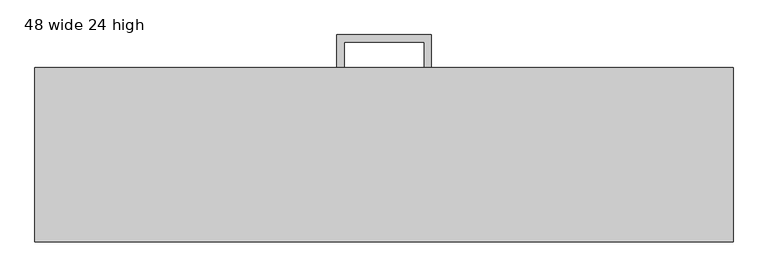
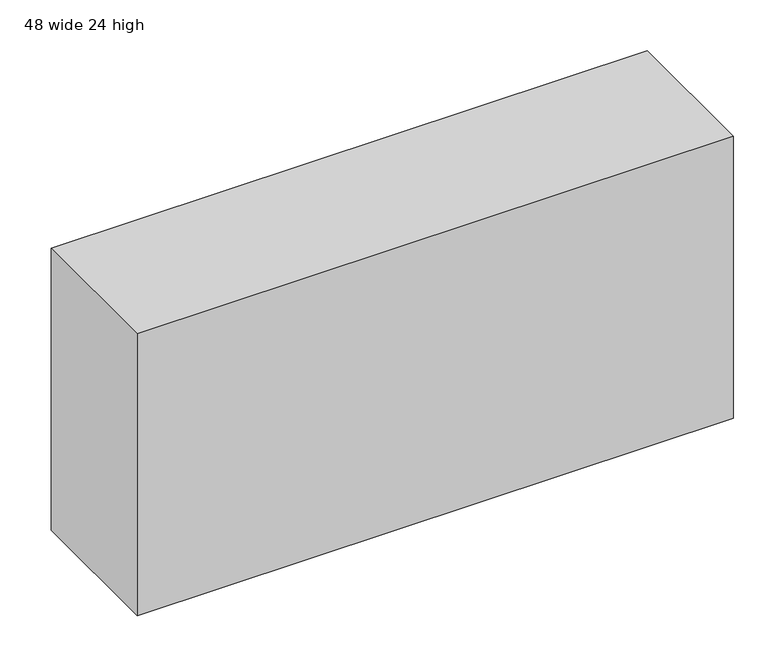
"""IFC4 building model written with IfcOpenShell, lengths in millimetres: furniture geometry, Binder Bin : 48 wide 24 high."""

from ifc_helpers import new_model, si_unit, frame, origin, place, context, project, spatial, polyline, outline, extrude, source, transform, mapped, element, save


def furniture_48_wide_24_high_fb19277b(model_context):
    return source(origin(), model_context, "Body", "SweptSolid", [
        extrude(outline(polyline([(-69.85, 381.0), (-82.55, 381.0), (-82.55, 438.15), (82.55, 438.15), (82.55, 381.0), (69.85, 381.0), (69.85, 425.45), (-69.85, 425.45), (-69.85, 381.0)])), frame((0.0, 0.0, 1416.05), z_axis=(0.0, 0.0, 1.0), x_axis=(1.0, 0.0, 0.0)), (0.0, 0.0, 1.0), 12.7),
        extrude(outline(polyline([(609.6, 76.2), (-609.6, 76.2), (-609.6, 381.0), (609.6, 381.0), (609.6, 76.2)])), frame((0.0, 0.0, 1371.6), z_axis=(0.0, 0.0, 1.0), x_axis=(1.0, 0.0, 0.0)), (0.0, 0.0, 1.0), 609.6),
    ])


if __name__ == "__main__":
    model = new_model("IFC4")
    model_context = context("Model", 3, world=origin())
    ifc_project = project(units=[si_unit("LENGTHUNIT", "METRE", prefix="MILLI")], contexts=[model_context])
    site = spatial("IfcSite", under=ifc_project)
    building = spatial("IfcBuilding", under=site)
    placement = place(None, origin())
    furniture_48_wide_24_high_shape = furniture_48_wide_24_high_fb19277b(model_context)
    element("IfcFurniture", 1, ObjectType="Binder Bin : 48 wide 24 high", at=placement, inside=building, context=model_context, shape_type="MappedRepresentation", body=[
        mapped(furniture_48_wide_24_high_shape, transform((0.0, 0.0, 0.0), x_axis=(1.0, 0.0, 0.0), y_axis=(0.0, 1.0, 0.0), z_axis=(0.0, 0.0, 1.0))),
    ])
    save(model, "model.ifc")

# Revit data of these elements
# Type "Binder Bin : 48 wide 24 high"
#   Model = "BIN-4824"
#   Manufacturer = "Corporate Concepts"
#   Type Mark = "BN-3"
#   Model = "BIN-4824"
#   Manufacturer = "Corporate Concepts"
#   Cost = 785
#   Width = 4' - 0"
#   Mounting Height [instance default] = 4' - 6"
#   Height = 2' - 0"
#   Cost = 785
#   Type Image = Binder Bin.png
#   Default Elevation = 0
